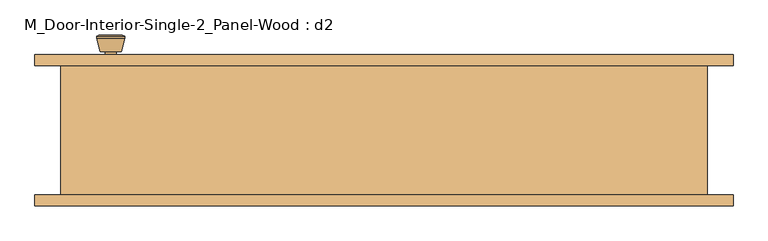
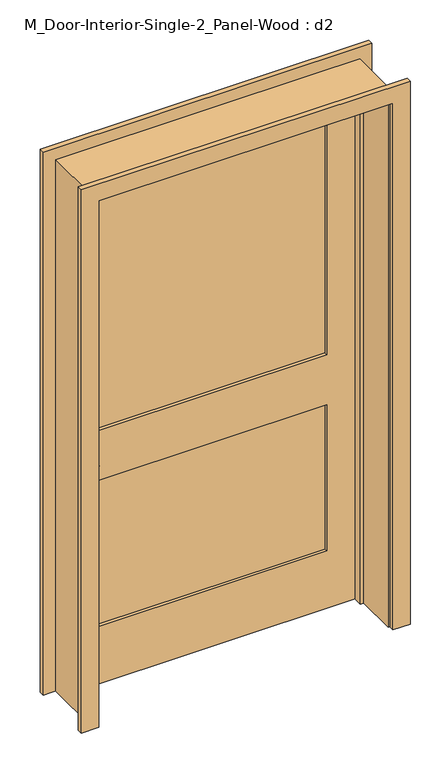
"""IFC4 building model written with IfcOpenShell, lengths in millimetres: door geometry, M_Door-Interior-Single-2_Panel-Wood : d2."""

import ifcopenshell
import ifcopenshell.guid

model = None  # the IFC model being written
_history = None  # IfcOwnerHistory: only IFC2X3 demands one
_inside = {}  # id of a spatial element -> (the spatial element, [elements in it])
_under = {}  # id of a project, library or spatial element -> (it, [spatial elements below it])
_declared = {}  # id of a project -> (the project, [libraries it declares])
_typed = {}  # id of a type object -> (the type object, [elements of that type])
_made_of = {}  # id of a material, layer set ... -> (it, [elements and type objects made of it])


def new_model(schema):
    """Start an empty IFC model of exactly this schema.

    Asked for "IFC4X3", IfcOpenShell would pick the latest addendum, in which some entities
    have other attributes; the version numbers below select the first issue.
    IFC2X3 requires an IfcOwnerHistory on every rooted entity: one is made here for all.
    """
    global model, _history
    if schema == "IFC4X3":
        model = ifcopenshell.file(schema_version=(4, 3, 0, 0))
    else:
        model = ifcopenshell.file(schema=schema)
    _inside.clear()
    _under.clear()
    _declared.clear()
    _typed.clear()
    _made_of.clear()
    _history = None
    if model.schema == "IFC2X3":
        org = make("IfcOrganization", Name="unknown")
        user = make(
            "IfcPersonAndOrganization",
            ThePerson=make("IfcPerson", FamilyName="unknown"),
            TheOrganization=org,
        )
        app = make(
            "IfcApplication",
            ApplicationDeveloper=org,
            Version="unknown",
            ApplicationFullName="unknown",
            ApplicationIdentifier="unknown",
        )
        _history = make(
            "IfcOwnerHistory",
            OwningUser=user,
            OwningApplication=app,
            ChangeAction="ADDED",
            CreationDate=0,
        )
    return model


def make(cls, **values):
    """One entity of the class cls with the attributes given. An attribute that is None is left unset."""
    return model.create_entity(
        cls, **{name: value for name, value in values.items() if value is not None}
    )


def rooted(cls, **values):
    """An entity with a GlobalId (a new one), such as an element, a storey or a relation."""
    return make(cls, GlobalId=ifcopenshell.guid.new(), OwnerHistory=_history, **values)


def si_unit(unit_type, name, prefix=None):
    """IfcSIUnit, for example si_unit("LENGTHUNIT", "METRE", prefix="MILLI")."""
    return make("IfcSIUnit", UnitType=unit_type, Prefix=prefix, Name=name)


def assignment(units):
    """IfcUnitAssignment: the units of a project."""
    return None if units is None else make("IfcUnitAssignment", Units=units)


def point(xyz):
    """IfcCartesianPoint."""
    return None if xyz is None else make("IfcCartesianPoint", Coordinates=xyz)


def direction(xyz):
    """IfcDirection."""
    return None if xyz is None else make("IfcDirection", DirectionRatios=xyz)


def frame(location, z_axis=None, x_axis=None):
    """IfcAxis2Placement3D, a coordinate frame: its origin and axes. An axis left out is left unset."""
    return make(
        "IfcAxis2Placement3D",
        Location=point(location),
        Axis=direction(z_axis),
        RefDirection=direction(x_axis),
    )


def frame_2d(location, x_axis=None):
    """IfcAxis2Placement2D, a coordinate frame in the plane: its origin and x axis."""
    return make(
        "IfcAxis2Placement2D", Location=point(location), RefDirection=direction(x_axis)
    )


def origin():
    """The frame at (0, 0, 0) with its axes left unset."""
    return frame((0.0, 0.0, 0.0))


def place(relative_to, where):
    """IfcLocalPlacement: puts the frame where relative to a parent placement (None: the world)."""
    return make(
        "IfcLocalPlacement", PlacementRelTo=relative_to, RelativePlacement=where
    )


def context(
    kind, dimensions, precision=None, world=None, true_north=None, identifier=None
):
    """IfcGeometricRepresentationContext, for example the 3D "Model" context."""
    return make(
        "IfcGeometricRepresentationContext",
        ContextIdentifier=identifier,
        ContextType=kind,
        CoordinateSpaceDimension=dimensions,
        Precision=precision,
        WorldCoordinateSystem=world,
        TrueNorth=true_north,
    )


def project(units=None, contexts=None):
    """IfcProject with its units and contexts."""
    return rooted(
        "IfcProject",
        Name="project",
        RepresentationContexts=contexts,
        UnitsInContext=assignment(units),
    )


def spatial(cls, under=None, at=None, **own):
    """A site, building, storey or space (cls), placed at a placement, below another one or the project."""
    s = rooted(cls, ObjectPlacement=at, **own)
    if under is not None:
        _under.setdefault(under.id(), (under, []))[1].append(s)
    return s


def polyline(points):
    """IfcPolyline through the points."""
    return make("IfcPolyline", Points=[point(p) for p in points])


def circle_curve(where, radius):
    """IfcCircle in the frame where."""
    return make("IfcCircle", Position=where, Radius=radius)


def trimmed(basis, trim1, trim2, sense, master):
    """IfcTrimmedCurve: the piece of a basis curve between two trims."""
    return make(
        "IfcTrimmedCurve",
        BasisCurve=basis,
        Trim1=trim1,
        Trim2=trim2,
        SenseAgreement=sense,
        MasterRepresentation=master,
    )


def segment(curve, same_sense, transition):
    """IfcCompositeCurveSegment."""
    return make(
        "IfcCompositeCurveSegment",
        Transition=transition,
        SameSense=same_sense,
        ParentCurve=curve,
    )


def composite_curve(segments, self_intersect=None):
    """IfcCompositeCurve: segments joined end to end."""
    return make("IfcCompositeCurve", Segments=segments, SelfIntersect=self_intersect)


def outline(outer, holes=None, kind="AREA"):
    """IfcArbitraryClosedProfileDef: a profile drawn as a closed curve; with holes, ...WithVoids."""
    if holes is None:
        return make("IfcArbitraryClosedProfileDef", ProfileType=kind, OuterCurve=outer)
    return make(
        "IfcArbitraryProfileDefWithVoids",
        ProfileType=kind,
        OuterCurve=outer,
        InnerCurves=holes,
    )


def extrude(swept, where, along, depth):
    """IfcExtrudedAreaSolid: the profile swept, set in the frame where, extruded along a direction by depth."""
    return make(
        "IfcExtrudedAreaSolid",
        SweptArea=swept,
        Position=where,
        ExtrudedDirection=direction(along),
        Depth=depth,
    )


def faces_of(points, faces, orient=None, outer=None):
    """IfcFace entities. A face is a list of loops; a loop is a list of indices into points, from 0.

    orient and outer hold one flag for each loop. By default every Orientation is true, the
    first loop of a face is its IfcFaceOuterBound and the others are IfcFaceBound.
    """
    made = []
    for i, loops in enumerate(faces):
        bounds = []
        for j, loop in enumerate(loops):
            is_outer = j == 0 if outer is None else outer[i][j]
            bounds.append(
                make(
                    "IfcFaceOuterBound" if is_outer else "IfcFaceBound",
                    Bound=make("IfcPolyLoop", Polygon=[points[k] for k in loop]),
                    Orientation=True if orient is None else orient[i][j],
                )
            )
        made.append(make("IfcFace", Bounds=bounds))
    return made


def faceted_brep(points, faces, orient=None, outer=None, voids=None):
    """IfcFacetedBrep: a solid bounded by flat faces; with voids (closed shells), ...WithVoids."""
    shared = [point(p) for p in points]
    hull = make("IfcClosedShell", CfsFaces=faces_of(shared, faces, orient, outer))
    if voids is None:
        return make("IfcFacetedBrep", Outer=hull)
    return make(
        "IfcFacetedBrepWithVoids",
        Outer=hull,
        Voids=[
            make(cls, CfsFaces=faces_of(shared, fs, o, b)) for cls, fs, o, b in voids
        ],
    )


def shape(context_of_items, identifier, shape_type, items):
    """IfcShapeRepresentation: the items that make up one representation, for example the "Body"."""
    return make(
        "IfcShapeRepresentation",
        ContextOfItems=context_of_items,
        RepresentationIdentifier=identifier,
        RepresentationType=shape_type,
        Items=items,
    )


def source(mapping_origin, context_of_items, identifier, shape_type, items):
    """IfcRepresentationMap: a shape defined once, which mapped items show again and again."""
    return make(
        "IfcRepresentationMap",
        MappingOrigin=mapping_origin,
        MappedRepresentation=shape(context_of_items, identifier, shape_type, items),
    )


def transform(
    local_origin,
    x_axis=None,
    y_axis=None,
    z_axis=None,
    scale=None,
    scale2=None,
    scale3=None,
    uniform=True,
):
    """IfcCartesianTransformationOperator3D, or its non-uniform kind. x_axis, y_axis, z_axis: its Axis1, 2, 3."""
    if uniform:
        return make(
            "IfcCartesianTransformationOperator3D",
            Axis1=direction(x_axis),
            Axis2=direction(y_axis),
            LocalOrigin=point(local_origin),
            Scale=scale,
            Axis3=direction(z_axis),
        )
    return make(
        "IfcCartesianTransformationOperator3DnonUniform",
        Axis1=direction(x_axis),
        Axis2=direction(y_axis),
        LocalOrigin=point(local_origin),
        Scale=scale,
        Axis3=direction(z_axis),
        Scale2=scale2,
        Scale3=scale3,
    )


def mapped(mapping_source, mapping_target):
    """IfcMappedItem: shows the shape of a source again, moved by a transform."""
    return make(
        "IfcMappedItem", MappingSource=mapping_source, MappingTarget=mapping_target
    )


def made_of(thing, what):
    """Note that an element or type object is made of a material, layer set ...; save() writes the relation."""
    if what is not None:
        _made_of.setdefault(what.id(), (what, []))[1].append(thing)
    return thing


def element(
    cls,
    number,
    at=None,
    inside=None,
    cuts=None,
    type_object=None,
    material=None,
    context=None,
    identifier="Body",
    shape_type=None,
    held_by="IfcProductDefinitionShape",
    body=None,
    shapes=None,
    **own,
):
    """One element of the class cls, such as IfcWall. Its Tag is "e" and its number.

    at: its placement. inside: the storey or other place that contains it. cuts: it is an
    opening in that element (IfcRelVoidsElement). A single representation is given by context,
    identifier, shape_type and body (its items); several are given by shapes. held_by: the class
    of the entity that holds the representations. save() writes the other relations.
    """
    e = rooted(cls, Tag="e%d" % number, ObjectPlacement=at, **own)
    if body is not None:
        shapes = [shape(context, identifier, shape_type, body)]
    if shapes is not None:
        e.Representation = make(held_by, Representations=shapes)
    if inside is not None:
        _inside.setdefault(inside.id(), (inside, []))[1].append(e)
    if cuts is not None:
        rooted(
            "IfcRelVoidsElement", RelatingBuildingElement=cuts, RelatedOpeningElement=e
        )
    if type_object is not None:
        _typed.setdefault(type_object.id(), (type_object, []))[1].append(e)
    return made_of(e, material)


def aggregate(whole, parts):
    """IfcRelAggregates: a whole, such as a stair, and the parts it consists of."""
    return rooted("IfcRelAggregates", RelatingObject=whole, RelatedObjects=parts)


def save(model, path):
    """Write the relations noted so far, then the file.

    IfcRelAggregates (storeys below a building ...), IfcRelContainedInSpatialStructure (elements
    in a storey), IfcRelDefinesByType, IfcRelAssociatesMaterial and IfcRelDeclares: one each for
    every whole, place, type object, material and project.
    """
    for whole, parts in _under.values():
        aggregate(whole, parts)
    for where, things in _inside.values():
        rooted(
            "IfcRelContainedInSpatialStructure",
            RelatedElements=things,
            RelatingStructure=where,
        )
    for kind, things in _typed.values():
        rooted("IfcRelDefinesByType", RelatedObjects=things, RelatingType=kind)
    for what, things in _made_of.values():
        rooted("IfcRelAssociatesMaterial", RelatedObjects=things, RelatingMaterial=what)
    for by, libraries in _declared.values():
        rooted("IfcRelDeclares", RelatingContext=by, RelatedDefinitions=libraries)
    model.write(path)


def plane_surface(at):
    """IfcPlane: the flat surface through the origin of the frame at, square to its z axis."""
    return make("IfcPlane", Position=at)


def cylinder_surface(at, radius):
    """IfcCylindricalSurface: all points at the distance radius from the z axis of the frame at."""
    return make("IfcCylindricalSurface", Position=at, Radius=radius)


def revolved_surface(curve, axis_point, axis_direction):
    """IfcSurfaceOfRevolution: the curve turned about the line through axis_point along axis_direction."""
    return make(
        "IfcSurfaceOfRevolution",
        SweptCurve=make("IfcArbitraryOpenProfileDef", ProfileType="CURVE", Curve=curve),
        AxisPosition=make("IfcAxis1Placement", Location=point(axis_point), Axis=direction(axis_direction)),
    )


def advanced_brep(points, edges, surfaces, faces):
    """IfcAdvancedBrep: a solid bounded by faces that lie on surfaces and meet in shared edges.

    An edge is (start, end): straight between two places in points (the first is 0);
    or (start, end, curve); or (start, end, curve, False) where it runs against its curve.
    A face is (place in surfaces, loops), or (place, loops, False) where it looks against
    its surface's normal. A loop lists edges by number (the first is 1), with a minus sign
    where the edge is run from its end to its start. The first loop is the outer one.
    """
    corners = [point(p) for p in points]
    vertices = [make("IfcVertexPoint", VertexGeometry=c) for c in corners]
    made = []
    for start, end, *more in edges:
        made.append(
            make(
                "IfcEdgeCurve",
                EdgeStart=vertices[start],
                EdgeEnd=vertices[end],
                EdgeGeometry=more[0] if more else make("IfcPolyline", Points=[corners[start], corners[end]]),
                SameSense=more[1] if len(more) > 1 else True,
            )
        )
    hull = []
    for where, loops, *sense in faces:
        bounds = []
        for j, loop in enumerate(loops):
            ring = [make("IfcOrientedEdge", EdgeElement=made[abs(k) - 1], Orientation=k > 0) for k in loop]
            bounds.append(
                make(
                    "IfcFaceOuterBound" if j == 0 else "IfcFaceBound",
                    Bound=make("IfcEdgeLoop", EdgeList=ring),
                    Orientation=True,
                )
            )
        hull.append(make("IfcAdvancedFace", Bounds=bounds, FaceSurface=surfaces[where], SameSense=sense[0] if sense else True))
    return make("IfcAdvancedBrep", Outer=make("IfcClosedShell", CfsFaces=hull))


def m_door_interior_single_2_panel_wood_d2_be971991(model_context):
    return source(origin(), model_context, "Body", "SolidModel", [
        advanced_brep(
        [(-486.5, 70.825, 914.4), (-476.5, 70.825, 914.4), (-496.5, 70.825, 914.4), (-466.0241324, 21.825, 914.4), (-486.5, 21.825, 914.4), (-506.9758676, 21.825, 914.4), (-461.5, 23.6528681, 914.4), (-511.5, 23.6528681, 914.4), (-461.5, 27.1165463, 914.4), (-511.5, 27.1165463, 914.4), (-467.863764, 51.825, 914.4), (-505.136236, 51.825, 914.4), (-476.5, 51.825, 914.4), (-496.5, 51.825, 914.4)],
        [
            (0, 1),
            (1, 2, circle_curve(frame((-486.5, 70.825, 914.4), z_axis=(0.0, 1.0, 0.0), x_axis=(-1.0, 0.0, 0.0)), 10.0)),
            (2, 0),
            (2, 1, circle_curve(frame((-486.5, 70.825, 914.4), z_axis=(0.0, 1.0, 0.0), x_axis=(-1.0, 0.0, 0.0)), 10.0)),
            (3, 4),
            (4, 5),
            (5, 3, circle_curve(frame((-486.5, 21.825, 914.4), z_axis=(0.0, -1.0, 0.0), x_axis=(-1.0, 0.0, 0.0)), 20.4758676)),
            (3, 5, circle_curve(frame((-486.5, 21.825, 914.4), z_axis=(0.0, -1.0, 0.0), x_axis=(-1.0, 0.0, 0.0)), 20.4758676)),
            (6, 3),
            (5, 7),
            (7, 6, circle_curve(frame((-486.5, 23.6528681, 914.4), z_axis=(0.0, -1.0, 0.0), x_axis=(-1.0, 0.0, 0.0)), 25.0)),
            (6, 7, circle_curve(frame((-486.5, 23.6528681, 914.4), z_axis=(0.0, -1.0, 0.0), x_axis=(-1.0, 0.0, 0.0)), 25.0)),
            (8, 6),
            (7, 9),
            (9, 8, circle_curve(frame((-486.5, 27.1165463, 914.4), z_axis=(0.0, -1.0, 0.0), x_axis=(-1.0, 0.0, 0.0)), 25.0)),
            (8, 9, circle_curve(frame((-486.5, 27.1165463, 914.4), z_axis=(0.0, -1.0, 0.0), x_axis=(-1.0, 0.0, 0.0)), 25.0)),
            (10, 8),
            (9, 11),
            (11, 10, circle_curve(frame((-486.5, 51.825, 914.4), z_axis=(0.0, -1.0, 0.0), x_axis=(-1.0, 0.0, 0.0)), 18.636236)),
            (10, 11, circle_curve(frame((-486.5, 51.825, 914.4), z_axis=(0.0, -1.0, 0.0), x_axis=(-1.0, 0.0, 0.0)), 18.636236)),
            (12, 10),
            (11, 13),
            (13, 12, circle_curve(frame((-486.5, 51.825, 914.4), z_axis=(0.0, -1.0, 0.0), x_axis=(-1.0, 0.0, 0.0)), 10.0)),
            (12, 13, circle_curve(frame((-486.5, 51.825, 914.4), z_axis=(0.0, -1.0, 0.0), x_axis=(-1.0, 0.0, 0.0)), 10.0)),
            (1, 12),
            (13, 2),
        ],
        [
            plane_surface(frame((-486.5, 70.825, 914.4), z_axis=(0.0, 1.0, 0.0), x_axis=(-1.0, 0.0, 0.0))),
            plane_surface(frame((-486.5, 21.825, 914.4), z_axis=(0.0, -1.0, 0.0), x_axis=(-1.0, 0.0, 0.0))),
            revolved_surface(polyline([(-506.9758676, 21.825, 914.4), (-511.5, 23.6528681, 914.4)]), (-486.5, 70.825, 914.4), (0.0, 1.0, 0.0)),
            cylinder_surface(frame((-486.5, 70.825, 914.4), z_axis=(0.0, 1.0, 0.0), x_axis=(-1.0, 0.0, 0.0)), 25.0),
            revolved_surface(polyline([(-511.5, 27.1165463, 914.4), (-505.136236, 51.825, 914.4)]), (-486.5, 70.825, 914.4), (0.0, 1.0, 0.0)),
            plane_surface(frame((-486.5, 51.825, 914.4), z_axis=(0.0, 1.0, 0.0), x_axis=(-1.0, 0.0, 0.0))),
            cylinder_surface(frame((-486.5, 70.825, 914.4), z_axis=(0.0, 1.0, 0.0), x_axis=(-1.0, 0.0, 0.0)), 10.0),
        ],
        [
            (0, [[1, 2, 3]]),
            (0, [[-3, 4, -1]]),
            (1, [[5, 6, 7]]),
            (1, [[-6, -5, 8]]),
            (2, [[9, -7, 10, 11]]),
            (2, [[-10, -8, -9, 12]]),
            (3, [[13, -11, 14, 15]]),
            (3, [[-14, -12, -13, 16]]),
            (4, [[17, -15, 18, 19]]),
            (4, [[-18, -16, -17, 20]]),
            (5, [[21, -19, 22, 23]]),
            (5, [[-22, -20, -21, 24]]),
            (6, [[25, -23, 26, -2]]),
            (6, [[-26, -24, -25, -4]]),
        ],
    ),
        extrude(outline(composite_curve([segment(trimmed(circle_curve(frame_2d((914.4, -486.5)), 30.0), [point((914.4, -516.5))], [point((914.4, -456.5))], False, "CARTESIAN"), True, "CONTINUOUS"), segment(trimmed(circle_curve(frame_2d((914.4, -486.5)), 30.0), [point((914.4, -456.5))], [point((914.4, -516.5))], False, "CARTESIAN"), True, "CONTINUOUS")], self_intersect=False)), frame((0.0, 70.825, 0.0), z_axis=(0.0, 1.0, 0.0), x_axis=(0.0, 0.0, 1.0)), (0.0, 0.0, 1.0), 6.0),
        advanced_brep(
        [(-486.5, 117.825, 914.4), (-496.5, 117.825, 914.4), (-476.5, 117.825, 914.4), (-466.0241324, 166.825, 914.4), (-506.9758676, 166.825, 914.4), (-486.5, 166.825, 914.4), (-461.5, 164.9971319, 914.4), (-511.5, 164.9971319, 914.4), (-461.5, 161.5334537, 914.4), (-511.5, 161.5334537, 914.4), (-467.863764, 136.825, 914.4), (-505.136236, 136.825, 914.4), (-476.5, 136.825, 914.4), (-496.5, 136.825, 914.4)],
        [
            (0, 1),
            (1, 2, circle_curve(frame((-486.5, 117.825, 914.4), z_axis=(0.0, -1.0, 0.0), x_axis=(-1.0, 0.0, 0.0)), 10.0)),
            (2, 0),
            (2, 1, circle_curve(frame((-486.5, 117.825, 914.4), z_axis=(0.0, -1.0, 0.0), x_axis=(-1.0, 0.0, 0.0)), 10.0)),
            (3, 4, circle_curve(frame((-486.5, 166.825, 914.4), z_axis=(0.0, 1.0, 0.0), x_axis=(-1.0, 0.0, 0.0)), 20.4758676)),
            (4, 5),
            (5, 3),
            (4, 3, circle_curve(frame((-486.5, 166.825, 914.4), z_axis=(0.0, 1.0, 0.0), x_axis=(-1.0, 0.0, 0.0)), 20.4758676)),
            (6, 7, circle_curve(frame((-486.5, 164.9971319, 914.4), z_axis=(0.0, 1.0, 0.0), x_axis=(-1.0, 0.0, 0.0)), 25.0)),
            (7, 4),
            (3, 6),
            (7, 6, circle_curve(frame((-486.5, 164.9971319, 914.4), z_axis=(0.0, 1.0, 0.0), x_axis=(-1.0, 0.0, 0.0)), 25.0)),
            (8, 9, circle_curve(frame((-486.5, 161.5334537, 914.4), z_axis=(0.0, 1.0, 0.0), x_axis=(-1.0, 0.0, 0.0)), 25.0)),
            (9, 7),
            (6, 8),
            (9, 8, circle_curve(frame((-486.5, 161.5334537, 914.4), z_axis=(0.0, 1.0, 0.0), x_axis=(-1.0, 0.0, 0.0)), 25.0)),
            (10, 11, circle_curve(frame((-486.5, 136.825, 914.4), z_axis=(0.0, 1.0, 0.0), x_axis=(-1.0, 0.0, 0.0)), 18.636236)),
            (11, 9),
            (8, 10),
            (11, 10, circle_curve(frame((-486.5, 136.825, 914.4), z_axis=(0.0, 1.0, 0.0), x_axis=(-1.0, 0.0, 0.0)), 18.636236)),
            (12, 13, circle_curve(frame((-486.5, 136.825, 914.4), z_axis=(0.0, 1.0, 0.0), x_axis=(-1.0, 0.0, 0.0)), 10.0)),
            (13, 11),
            (10, 12),
            (13, 12, circle_curve(frame((-486.5, 136.825, 914.4), z_axis=(0.0, 1.0, 0.0), x_axis=(-1.0, 0.0, 0.0)), 10.0)),
            (1, 13),
            (12, 2),
        ],
        [
            plane_surface(frame((-486.5, 117.825, 914.4), z_axis=(0.0, -1.0, 0.0), x_axis=(-1.0, 0.0, 0.0))),
            plane_surface(frame((-486.5, 166.825, 914.4), z_axis=(0.0, 1.0, 0.0), x_axis=(-1.0, 0.0, 0.0))),
            revolved_surface(polyline([(-506.9758676, 166.825, 914.4), (-511.5, 164.9971319, 914.4)]), (-486.5, 117.825, 914.4), (0.0, -1.0, 0.0)),
            cylinder_surface(frame((-486.5, 117.825, 914.4), z_axis=(0.0, -1.0, 0.0), x_axis=(-1.0, 0.0, 0.0)), 25.0),
            revolved_surface(polyline([(-511.5, 161.5334537, 914.4), (-505.136236, 136.825, 914.4)]), (-486.5, 117.825, 914.4), (0.0, -1.0, 0.0)),
            plane_surface(frame((-486.5, 136.825, 914.4), z_axis=(0.0, -1.0, 0.0), x_axis=(-1.0, 0.0, 0.0))),
            cylinder_surface(frame((-486.5, 117.825, 914.4), z_axis=(0.0, -1.0, 0.0), x_axis=(-1.0, 0.0, 0.0)), 10.0),
        ],
        [
            (0, [[1, 2, 3]]),
            (0, [[-3, 4, -1]]),
            (1, [[5, 6, 7]]),
            (1, [[8, -7, -6]]),
            (2, [[9, 10, -5, 11]]),
            (2, [[12, -11, -8, -10]]),
            (3, [[13, 14, -9, 15]]),
            (3, [[16, -15, -12, -14]]),
            (4, [[17, 18, -13, 19]]),
            (4, [[20, -19, -16, -18]]),
            (5, [[21, 22, -17, 23]]),
            (5, [[24, -23, -20, -22]]),
            (6, [[-2, 25, -21, 26]]),
            (6, [[-4, -26, -24, -25]]),
        ],
    ),
        extrude(outline(composite_curve([segment(trimmed(circle_curve(frame_2d((914.4, -486.5)), 30.0), [point((914.4, -516.5))], [point((914.4, -456.5))], False, "CARTESIAN"), True, "CONTINUOUS"), segment(trimmed(circle_curve(frame_2d((914.4, -486.5)), 30.0), [point((914.4, -456.5))], [point((914.4, -516.5))], False, "CARTESIAN"), True, "CONTINUOUS")], self_intersect=False)), frame((0.0, 111.825, 0.0), z_axis=(0.0, 1.0, 0.0), x_axis=(0.0, 0.0, 1.0)), (0.0, 0.0, 1.0), 6.0),
        extrude(outline(polyline([(430.0, 88.4916667), (-430.0, 88.4916667), (-430.0, 100.1583333), (430.0, 100.1583333), (430.0, 88.4916667)])), frame((0.0, 0.0, 1014.4), z_axis=(0.0, 0.0, 1.0), x_axis=(1.0, 0.0, 0.0)), (0.0, 0.0, 1.0), 965.6),
        extrude(outline(polyline([(430.0, 88.4916667), (-430.0, 88.4916667), (-430.0, 100.1583333), (430.0, 100.1583333), (430.0, 88.4916667)])), frame((0.0, 0.0, 230.0), z_axis=(0.0, 0.0, 1.0), x_axis=(1.0, 0.0, 0.0)), (0.0, 0.0, 1.0), 584.4),
        extrude(outline(polyline([(2100.0, -550.0), (0.0, -550.0), (0.0, 550.0), (2100.0, 550.0), (2100.0, -550.0)]), holes=[polyline([(1980.0, -430.0), (1980.0, 430.0), (1014.4, 430.0), (1014.4, -430.0), (1980.0, -430.0)]), polyline([(814.4, -430.0), (814.4, 430.0), (230.0, 430.0), (230.0, -430.0), (814.4, -430.0)])]), frame((0.0, 76.825, 0.0), z_axis=(0.0, 1.0, 0.0), x_axis=(0.0, 0.0, 1.0)), (0.0, 0.0, 1.0), 35.0),
        faceted_brep([(575.0, 111.825, 0.0), (575.0, -118.175, 0.0), (550.0, -118.175, 0.0), (550.0, 41.9, 0.0), (537.3, 41.9, 0.0), (537.3, 76.825, 0.0), (550.0, 76.825, 0.0), (550.0, 111.825, 0.0), (575.0, 111.825, 2125.0), (575.0, -118.175, 2125.0), (-575.0, -118.175, 2125.0), (-575.0, -118.175, 0.0), (-550.0, -118.175, 0.0), (-550.0, -118.175, 2100.0), (550.0, -118.175, 2100.0), (550.0, 41.9, 2100.0), (-550.0, 41.9, 2100.0), (-550.0, 41.9, 0.0), (-537.3, 41.9, 0.0), (-537.3, 41.9, 2087.3), (537.3, 41.9, 2087.3), (537.3, 76.825, 2087.3), (-537.3, 76.825, 2087.3), (-537.3, 76.825, 0.0), (-550.0, 76.825, 0.0), (-550.0, 76.825, 2100.0), (550.0, 76.825, 2100.0), (550.0, 111.825, 2100.0), (-550.0, 111.825, 2100.0), (-550.0, 111.825, 0.0), (-575.0, 111.825, 0.0), (-575.0, 111.825, 2125.0)], [[[0, 1, 2, 3, 4, 5, 6, 7]], [[1, 0, 8, 9]], [[2, 1, 9, 10, 11, 12, 13, 14]], [[3, 2, 14, 15]], [[4, 3, 15, 16, 17, 18, 19, 20]], [[5, 4, 20, 21]], [[6, 5, 21, 22, 23, 24, 25, 26]], [[7, 6, 26, 27]], [[0, 7, 27, 28, 29, 30, 31, 8]], [[9, 8, 31, 10]], [[15, 14, 13, 16]], [[21, 20, 19, 22]], [[27, 26, 25, 28]], [[30, 29, 24, 23, 18, 17, 12, 11]], [[10, 31, 30, 11]], [[16, 13, 12, 17]], [[22, 19, 18, 23]], [[28, 25, 24, 29]]]),
        extrude(outline(polyline([(0.0, 556.35), (0.0, 621.35), (2171.35, 621.35), (2171.35, -621.35), (0.0, -621.35), (0.0, -556.35), (2106.35, -556.35), (2106.35, 556.35), (0.0, 556.35)])), frame((0.0, -138.175, 0.0), z_axis=(0.0, 1.0, 0.0), x_axis=(0.0, 0.0, 1.0)), (0.0, 0.0, 1.0), 20.0),
        extrude(outline(polyline([(0.0, 556.35), (0.0, 621.35), (2171.35, 621.35), (2171.35, -621.35), (0.0, -621.35), (0.0, -556.35), (2106.35, -556.35), (2106.35, 556.35), (0.0, 556.35)])), frame((0.0, 111.825, 0.0), z_axis=(0.0, 1.0, 0.0), x_axis=(0.0, 0.0, 1.0)), (0.0, 0.0, 1.0), 20.0),
    ])


if __name__ == "__main__":
    model = new_model("IFC4")
    model_context = context("Model", 3, world=origin())
    ifc_project = project(units=[si_unit("LENGTHUNIT", "METRE", prefix="MILLI")], contexts=[model_context])
    site = spatial("IfcSite", under=ifc_project)
    building = spatial("IfcBuilding", under=site)
    placement = place(None, origin())
    m_door_interior_single_2_panel_wood_d2_shape = m_door_interior_single_2_panel_wood_d2_be971991(model_context)
    element("IfcDoor", 1, ObjectType="M_Door-Interior-Single-2_Panel-Wood : d2", at=placement, inside=building, context=model_context, shape_type="MappedRepresentation", body=[
        mapped(m_door_interior_single_2_panel_wood_d2_shape, transform((0.0, 0.0, 0.0), x_axis=(1.0, 0.0, 0.0), y_axis=(0.0, 1.0, 0.0), z_axis=(0.0, 0.0, 1.0))),
    ])
    save(model, "model.ifc")

# Revit data of these elements
# Type "M_Door-Interior-Single-2_Panel-Wood : d2"
#   Type Mark = "53"
#   Assembly Code = "C1020300"
#   Analytic Construction = "Wooden"
#   Top Rail = 12 cm
#   Thickness = 3.5 cm
#   Thermal Resistance (R) = 0.455703 (m²·K)/W
#   Swing Angle [instance default] = 90.00°
#   Stiles = 12 cm
#   Rough Width = 115 cm
#   Rough Height = 212.5 cm
#   Lock Rail = 20 cm
#   Height = 210 cm
#   Width = 110 cm
#   Heat Transfer Coefficient (U) = 2.19465 W/(m²·K)
#   Bottom Rail = 23 cm
#   Trim Material = Cherry
#   Panel Material = Cherry
#   Frame Material = Cherry
#   Door Handle Material = Aluminum
#   Visual Light Transmittance = 0
#   Solar Heat Gain Coefficient = 0
#   Wall Closure = (empty or 0)
#   Function = (empty or 0)
# Element 1 (IfcDoor, "M_Door-Interior-Single-2_Panel-Wood : d2")
#   Materials on its faces: "Cherry", "Aluminum"
# Materials
#   "Cherry": class "Wood", colour RGB 226 177 128, transparency 0, Description = "Prunus Serotina", Cost = 0
#   "Aluminum": class "Metal", colour RGB 247 247 247, transparency 0, Description = "Aluminum 6061", Cost = 0
